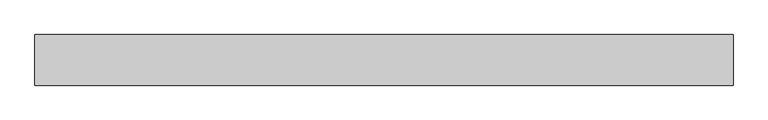
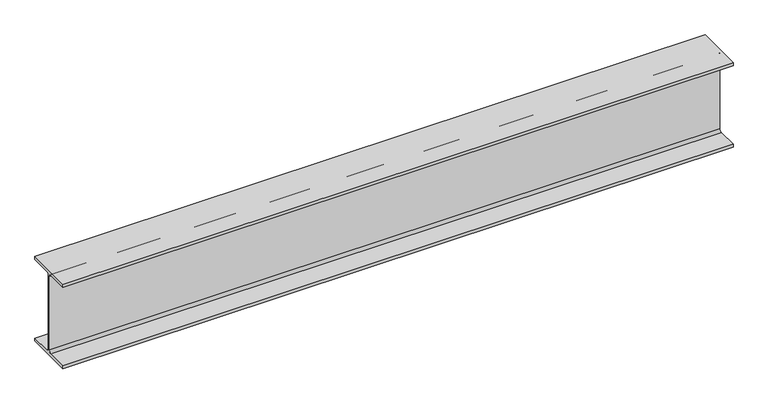
"""IFC4 building model written with IfcOpenShell, lengths in millimetres: beam geometry, Old_Steel Beam_H-KSD3502 : H_SB_ASB_H-200×200x8x12."""

from ifc_helpers import new_model, si_unit, point, frame, frame_2d, origin, place, context, project, spatial, polyline, circle_curve, trimmed, segment, composite_curve, outline, extrude, source, transform, mapped, element, save


def beam_8c5619d4(model_context):
    return source(origin(), model_context, "Body", "SweptSolid", [
        extrude(outline(composite_curve([segment(polyline([(82.5, -141.5), (82.5, -151.7), (-82.5, -151.7), (-82.5, -141.5), (-11.9, -141.5)]), True, "CONTINUOUS"), segment(trimmed(circle_curve(frame_2d((-11.9, -132.6)), 8.9), [point((-11.9, -141.5))], [point((-3.0, -132.6))], True, "CARTESIAN"), True, "CONTINUOUS"), segment(polyline([(-3.0, -132.6), (-3.0, 132.6)]), True, "CONTINUOUS"), segment(trimmed(circle_curve(frame_2d((-11.9, 132.6)), 8.9), [point((-3.0, 132.6))], [point((-11.9, 141.5))], True, "CARTESIAN"), True, "CONTINUOUS"), segment(polyline([(-11.9, 141.5), (-82.5, 141.5), (-82.5, 151.7), (82.5, 151.7), (82.5, 141.5), (11.9, 141.5)]), True, "CONTINUOUS"), segment(trimmed(circle_curve(frame_2d((11.9, 132.6)), 8.9), [point((11.9, 141.5))], [point((3.0, 132.6))], True, "CARTESIAN"), True, "CONTINUOUS"), segment(polyline([(3.0, 132.6), (3.0, -132.6)]), True, "CONTINUOUS"), segment(trimmed(circle_curve(frame_2d((11.9, -132.6)), 8.9), [point((3.0, -132.6))], [point((11.9, -141.5))], True, "CARTESIAN"), True, "CONTINUOUS"), segment(polyline([(11.9, -141.5), (82.5, -141.5)]), True, "CONTINUOUS")], self_intersect=False)), frame((-1039.9887612, 0.0, 0.0), z_axis=(1.0, 0.0, 0.0), x_axis=(0.0, 1.0, 0.0)), (0.0, 0.0, 1.0), 2275.0622856),
    ])


if __name__ == "__main__":
    model = new_model("IFC4")
    model_context = context("Model", 3, world=origin())
    ifc_project = project(units=[si_unit("LENGTHUNIT", "METRE", prefix="MILLI")], contexts=[model_context])
    site = spatial("IfcSite", under=ifc_project)
    building = spatial("IfcBuilding", under=site)
    placement = place(None, origin())
    beam_shape = beam_8c5619d4(model_context)
    element("IfcBeam", 1, ObjectType="Old_Steel Beam_H-KSD3502 : H_SB_ASB_H-200×200x8x12", at=placement, inside=building, context=model_context, shape_type="MappedRepresentation", body=[
        mapped(beam_shape, transform((0.0, 0.0, 0.0), x_axis=(1.0, 0.0, 0.0), y_axis=(0.0, 1.0, 0.0), z_axis=(0.0, 0.0, 1.0))),
    ])
    save(model, "model.ifc")

# Revit data of these elements
# Type "Old_Steel Beam_H-KSD3502 : H_SB_ASB_H-200×200x8x12"
#   Width = 20.0 cm
#   Web Thickness = 0.8 cm
#   Web Fillet = 1.3 cm
#   Warping Constant = 141376.0 cm⁶
#   Torsional Moment of Inertia = 26.2485 cm⁴
#   Torsional Modulus = 1.0 cm³
#   Section Area = 63.53 cm²
#   Plastic Modulus weak axis = 244.0 cm³
#   Plastic Modulus strong axis = 525.0 cm³
#   Perimeter = 1.16 m²/m
#   Nominal Weight = 49.90 kgf/m
#   Moment of Inertia weak axis = 1600.00 cm⁴
#   Moment of Inertia strong axis = 4720.00 cm⁴
#   Height = 20.0 cm
#   Flange Thickness = 1.2 cm
#   Elastic Modulus weak axis = 160.0 cm³
#   Elastic Modulus strong axis = 472.0 cm³
#   Centroid Vertical = 10.0 cm
#   Centroid Horizontal = 10.0 cm
#   Length [instance default] = 1.5240 m
#   Structural Material [instance default] = Steel, 45-345
#   Assembly Code = ""
# Element 1 (IfcBeam, "Old_Steel Beam_H-KSD3502 : H_SB_ASB_H-200×200x8x12")
#   Structural Material = none
# Materials
#   "Steel, 45-345": class "Metal", colour RGB 189 187 185, transparency 0, Description = "Steel 345 MPa", Cost = 0
